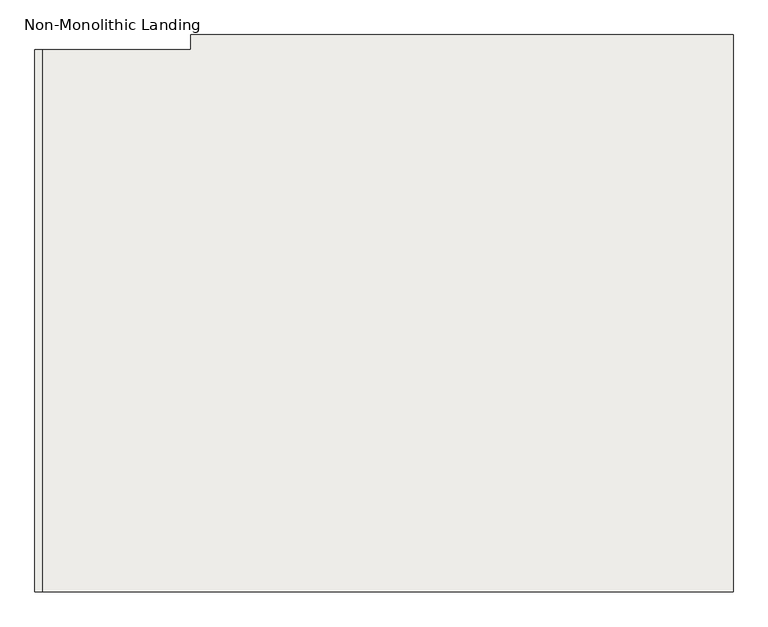
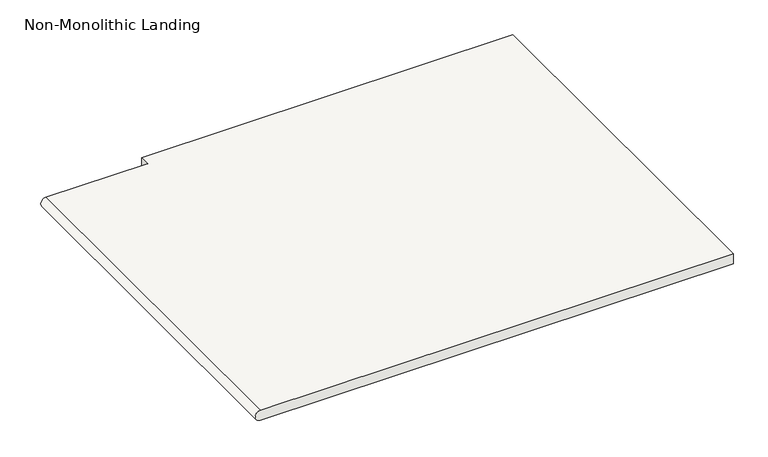
"""IFC4 building model written with IfcOpenShell, lengths in millimetres: slab geometry, Non-Monolithic Landing."""

from ifc_helpers import new_model, si_unit, frame, origin, place, context, project, spatial, circle_curve, source, transform, mapped, element, save
from ifc_brep_helpers import plane_surface, cylinder_surface, advanced_brep


def non_monolithic_landing_3de38245(model_context):
    return source(origin(), model_context, "Body", "AdvancedBrep", [
        advanced_brep(
        [(6239.7741968, -13363.3557429, 1689.1), (6239.7741968, -13363.3557429, 1714.5), (6239.7741968, -12448.9557429, 1714.5), (6239.7741968, -12448.9557429, 1689.1), (7404.2789345, -13363.3557429, 1714.5), (7404.2789345, -12448.9557429, 1714.5), (7404.2789345, -12423.5557429, 1714.5), (6489.8789345, -12423.5557429, 1714.5), (6489.8789345, -12448.9557429, 1714.5), (7404.2789345, -13363.3557429, 1689.1), (6489.8789345, -12448.9557429, 1689.1), (6489.8789345, -12423.5557429, 1689.1), (7404.2789345, -12423.5557429, 1689.1), (7404.2789345, -12448.9557429, 1689.1)],
        [
            (0, 1, circle_curve(frame((6239.7741968, -13363.3557429, 1701.8), z_axis=(0.0, 1.0, 0.0), x_axis=(1.0, 0.0, 0.0)), 12.7)),
            (1, 2),
            (2, 3, circle_curve(frame((6239.7741968, -12448.9557429, 1701.8), z_axis=(0.0, -1.0, 0.0), x_axis=(1.0, 0.0, 0.0)), 12.7)),
            (3, 0),
            (1, 4),
            (4, 5),
            (5, 6),
            (6, 7),
            (7, 8),
            (8, 2),
            (9, 0),
            (3, 10),
            (10, 11),
            (11, 12),
            (12, 13),
            (13, 9),
            (9, 4),
            (13, 5),
            (12, 6),
            (11, 7),
            (10, 8),
        ],
        [
            cylinder_surface(frame((6239.7741968, -13363.3557429, 1701.8), z_axis=(0.0, -1.0, 0.0), x_axis=(1.0, 0.0, 0.0)), 12.7),
            plane_surface(frame((6239.7741968, -12448.9557429, 1714.5), z_axis=(0.0, 0.0, 1.0), x_axis=(0.0, -1.0, 0.0))),
            plane_surface(frame((6239.7741968, -12448.9557429, 1689.1), z_axis=(0.0, 0.0, -1.0), x_axis=(0.0, 1.0, 0.0))),
            plane_surface(frame((6239.7741968, -13363.3557429, 1714.5), z_axis=(0.0, -1.0, 0.0), x_axis=(0.0, 0.0, -1.0))),
            plane_surface(frame((7404.2789345, -13363.3557429, 1714.5), z_axis=(1.0, 0.0, 0.0), x_axis=(0.0, 0.0, -1.0))),
            plane_surface(frame((7404.2789345, -12448.9557429, 1714.5), z_axis=(1.0, 0.0, 0.0), x_axis=(0.0, 0.0, -1.0))),
            plane_surface(frame((7404.2789345, -12423.5557429, 1714.5), z_axis=(0.0, 1.0, 0.0), x_axis=(0.0, 0.0, -1.0))),
            plane_surface(frame((6489.8789345, -12423.5557429, 1714.5), z_axis=(-1.0, 0.0, 0.0), x_axis=(0.0, 0.0, -1.0))),
            plane_surface(frame((6489.8789345, -12448.9557429, 1714.5), z_axis=(0.0, 1.0, 0.0), x_axis=(0.0, 0.0, -1.0))),
        ],
        [
            (0, [[1, 2, 3, 4]]),
            (1, [[5, 6, 7, 8, 9, 10, -2]]),
            (2, [[11, -4, 12, 13, 14, 15, 16]]),
            (3, [[-5, -1, -11, 17]]),
            (4, [[-6, -17, -16, 18]]),
            (5, [[-7, -18, -15, 19]]),
            (6, [[-8, -19, -14, 20]]),
            (7, [[-9, -20, -13, 21]]),
            (8, [[-10, -21, -12, -3]]),
        ],
    ),
    ])


if __name__ == "__main__":
    model = new_model("IFC4")
    model_context = context("Model", 3, world=origin())
    ifc_project = project(units=[si_unit("LENGTHUNIT", "METRE", prefix="MILLI")], contexts=[model_context])
    site = spatial("IfcSite", under=ifc_project)
    building = spatial("IfcBuilding", under=site)
    placement = place(None, origin())
    non_monolithic_landing_shape = non_monolithic_landing_3de38245(model_context)
    element("IfcSlab", 1, ObjectType="Non-Monolithic Landing", at=placement, inside=building, context=model_context, shape_type="MappedRepresentation", body=[
        mapped(non_monolithic_landing_shape, transform((0.0, 0.0, 0.0), x_axis=(1.0, 0.0, 0.0), y_axis=(0.0, 1.0, 0.0), z_axis=(0.0, 0.0, 1.0))),
    ])
    save(model, "model.ifc")

# Revit data of these elements
# Element 1 (IfcSlab, "Non-Monolithic Landing")
#   Materials on its faces: "Cherry"
# Materials
#   "Cherry": class "Wood", colour RGB 233 182 144, transparency 0, Description = "Prunus Serotina", Cost = 0
